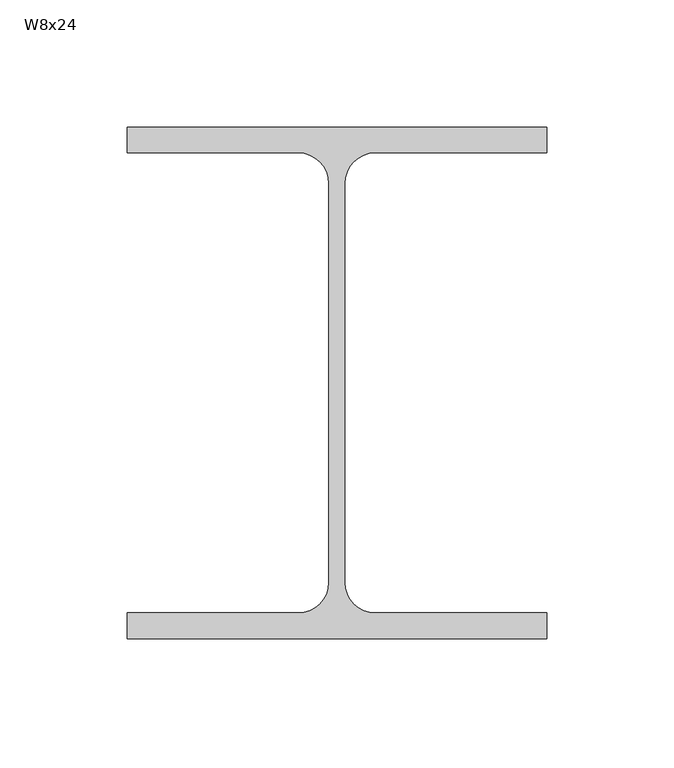
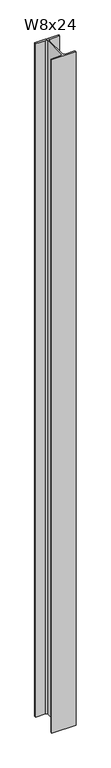
"""IFC4 building model written with IfcOpenShell, lengths in millimetres: column geometry, RME WF - Column : W8x24."""

from ifc_helpers import new_model, si_unit, point, frame, frame_2d, origin, place, context, project, spatial, polyline, circle_curve, trimmed, segment, composite_curve, outline, extrude, source, transform, mapped, element, save


def w8x24_2a02c570(model_context):
    return source(origin(), model_context, "Body", "SweptSolid", [
        extrude(outline(composite_curve([segment(polyline([(82.55, 100.711), (82.55, 90.551), (15.1765, 90.551)]), True, "CONTINUOUS"), segment(trimmed(circle_curve(frame_2d((15.1765, 78.486)), 12.065), [point((15.1765, 90.551))], [point((3.1115, 78.486))], True, "CARTESIAN"), True, "CONTINUOUS"), segment(polyline([(3.1115, 78.486), (3.1115, -78.486)]), True, "CONTINUOUS"), segment(trimmed(circle_curve(frame_2d((15.1765, -78.486)), 12.065), [point((3.1115, -78.486))], [point((15.1765, -90.551))], True, "CARTESIAN"), True, "CONTINUOUS"), segment(polyline([(15.1765, -90.551), (82.55, -90.551), (82.55, -100.711), (-82.55, -100.711), (-82.55, -90.551), (-15.1765, -90.551)]), True, "CONTINUOUS"), segment(trimmed(circle_curve(frame_2d((-15.1765, -78.486)), 12.065), [point((-15.1765, -90.551))], [point((-3.1115, -78.486))], True, "CARTESIAN"), True, "CONTINUOUS"), segment(polyline([(-3.1115, -78.486), (-3.1115, 78.486)]), True, "CONTINUOUS"), segment(trimmed(circle_curve(frame_2d((-15.1765, 78.486)), 12.065), [point((-3.1115, 78.486))], [point((-15.1765, 90.551))], True, "CARTESIAN"), True, "CONTINUOUS"), segment(polyline([(-15.1765, 90.551), (-82.55, 90.551), (-82.55, 100.711), (82.55, 100.711)]), True, "CONTINUOUS")], self_intersect=False)), frame((0.0, 0.0, -304.8), z_axis=(0.0, 0.0, 1.0), x_axis=(1.0, 0.0, 0.0)), (0.0, 0.0, 1.0), 4854.575),
    ])


if __name__ == "__main__":
    model = new_model("IFC4")
    model_context = context("Model", 3, world=origin())
    ifc_project = project(units=[si_unit("LENGTHUNIT", "METRE", prefix="MILLI")], contexts=[model_context])
    site = spatial("IfcSite", under=ifc_project)
    building = spatial("IfcBuilding", under=site)
    placement = place(None, origin())
    w8x24_shape = w8x24_2a02c570(model_context)
    element("IfcColumn", 1, ObjectType="RME WF - Column : W8x24", at=placement, inside=building, context=model_context, shape_type="MappedRepresentation", body=[
        mapped(w8x24_shape, transform((0.0, 0.0, 0.0), x_axis=(1.0, 0.0, 0.0), y_axis=(0.0, 1.0, 0.0), z_axis=(0.0, 0.0, 1.0))),
    ])
    save(model, "model.ifc")

# Revit data of these elements
# Type "RME WF - Column : W8x24"
#   Type Mark = "C1"
#   REINF TYPE [instance default] = ""
#   Nominal Size = "W16"
#   COL REMARKS [instance default] = ""
#   BP [instance default] = ""
#   Assembly Code = "B10"
#   W = 24
#   bf = 0' - 6 1/2"
#   d = 0' - 7.93"
#   k = 0' - 0 7/8"
#   kr = 0' - 0.475"
#   tf = 0' - 0.4"
#   tw = 0' - 0.245"
#   A = 0.0491667 SF
#   Structural Material [instance default] = Metal - Steel - ASTM A992
# Element 1 (IfcColumn, "RME WF - Column : W8x24")
#   Materials on its faces: "Metal - Steel - ASTM A992"
# Materials
#   "Metal - Steel - ASTM A992": class "Metal", colour RGB 255 128 0, transparency 0
